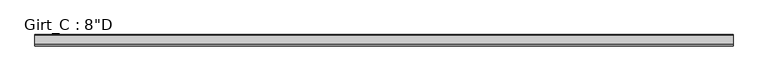
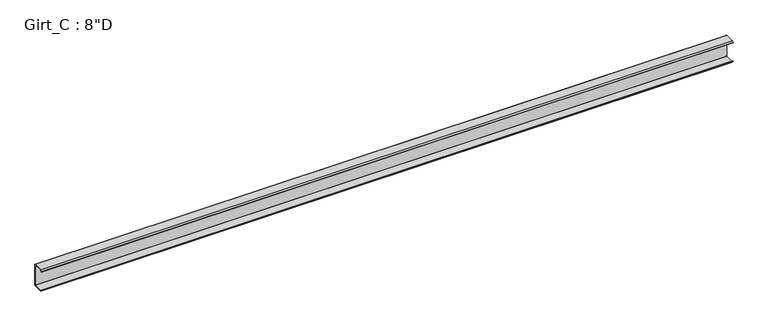
"""IFC4 building model written with IfcOpenShell, lengths in millimetres: beam geometry."""

from ifc_helpers import new_model, si_unit, point, frame, frame_2d, origin, place, context, project, spatial, polyline, circle_curve, trimmed, segment, composite_curve, outline, extrude, source, transform, mapped, element, save


def beam_00c11b00(model_context):
    return source(origin(), model_context, "Body", "SweptSolid", [
        extrude(outline(composite_curve([segment(polyline([(-87.5109375, 101.6), (-3.3734375, 101.6)]), True, "CONTINUOUS"), segment(trimmed(circle_curve(frame_2d((-3.3734375, 96.8375)), 4.7625), [point((-3.3734375, 101.6))], [point((1.3890625, 96.8375))], False, "CARTESIAN"), True, "CONTINUOUS"), segment(polyline([(1.3890625, 96.8375), (1.3890625, -96.8375)]), True, "CONTINUOUS"), segment(trimmed(circle_curve(frame_2d((-3.3734375, -96.8375)), 4.7625), [point((1.3890625, -96.8375))], [point((-3.3734375, -101.6))], False, "CARTESIAN"), True, "CONTINUOUS"), segment(polyline([(-3.3734375, -101.6), (-87.5109375, -101.6), (-99.7792647, -86.979177), (-97.6510975, -85.1934327), (-86.2154765, -98.821875), (-3.2694106, -98.821875)]), True, "CONTINUOUS"), segment(trimmed(circle_curve(frame_2d((-3.3748024, -96.8389339)), 1.9857399), [point((-3.2694106, -98.821875))], [point((-1.3890625, -96.8389339))], True, "CARTESIAN"), True, "CONTINUOUS"), segment(polyline([(-1.3890625, -96.8389339), (-1.3890625, 96.8381931)]), True, "CONTINUOUS"), segment(trimmed(circle_curve(frame_2d((-3.3741066, 96.8381931)), 1.9850441), [point((-1.3890625, 96.8381931))], [point((-3.3005807, 98.821875))], True, "CARTESIAN"), True, "CONTINUOUS"), segment(polyline([(-3.3005807, 98.821875), (-86.2154765, 98.821875), (-97.6278742, 85.221109), (-99.7560415, 87.0068534), (-87.5109375, 101.6)]), True, "CONTINUOUS")], self_intersect=False)), frame((-3100.3875, 0.0, 0.0), z_axis=(1.0, 0.0, 0.0), x_axis=(0.0, 1.0, 0.0)), (0.0, 0.0, 1.0), 6200.775),
    ])


if __name__ == "__main__":
    model = new_model("IFC4")
    model_context = context("Model", 3, world=origin())
    ifc_project = project(units=[si_unit("LENGTHUNIT", "METRE", prefix="MILLI")], contexts=[model_context])
    site = spatial("IfcSite", under=ifc_project)
    building = spatial("IfcBuilding", under=site)
    placement = place(None, origin())
    beam_shape = beam_00c11b00(model_context)
    element("IfcBeam", 1, ObjectType="Girt_C : 8\"D", at=placement, inside=building, context=model_context, shape_type="MappedRepresentation", body=[
        mapped(beam_shape, transform((0.0, 0.0, 0.0), x_axis=(1.0, 0.0, 0.0), y_axis=(0.0, 1.0, 0.0), z_axis=(0.0, 0.0, 1.0))),
    ])
    save(model, "model.ifc")

# Revit data of these elements
# Type "Girt_C : 8\"D"
#   half leg = 0' - 1 3/4"
#   Web_Thickness = 0' - 0 7/64"
#   Length [instance default] = 10' - 0"
#   Leg_1 = 0' - 3 1/2"
#   Height = 0' - 8"
#   Structural Material [instance default] = none
# Element 1 (IfcBeam, "Girt_C : 8\"D")
#   Structural Material = CEE' SECTION (8.0x3.5C - SEE STRUCT. DWGS)
#   Materials on its faces: "CEE' SECTION (8.0x3.5C - SEE STRUCT. DWGS)"
# Materials
#   "CEE' SECTION (8.0x3.5C - SEE STRUCT. DWGS)": class "Metal", colour RGB 137 146 153, transparency 0, Description = "Steel, mill finish", Cost = 0
